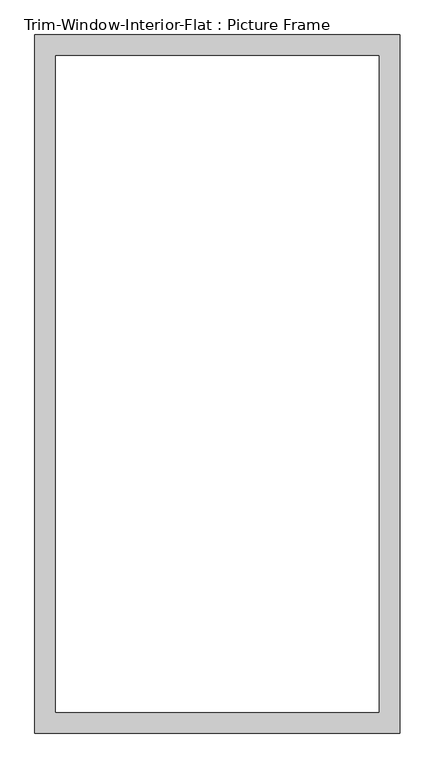
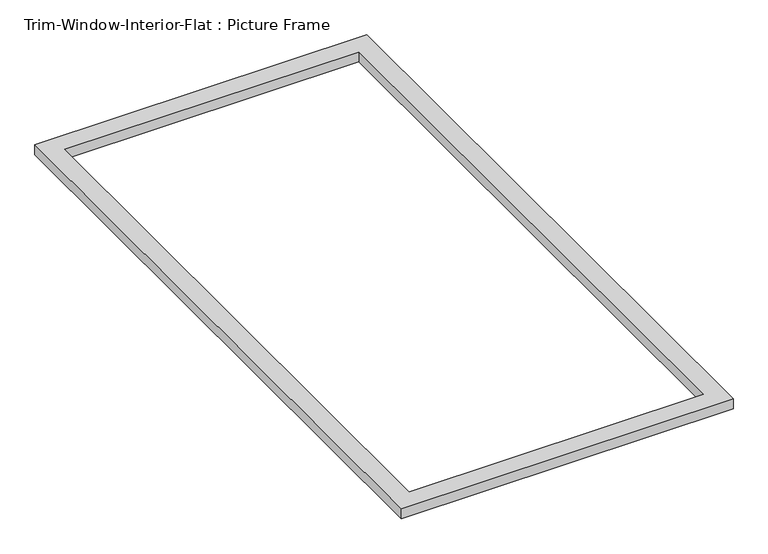
"""IFC4 building model written with IfcOpenShell, lengths in millimetres: proxy geometry, Trim-Window-Interior-Flat : Picture Frame."""

from ifc_helpers import new_model, si_unit, origin, origin_with_axes, place, context, project, spatial, polyline, outline, extrude, source, transform, mapped, element, save


def trim_window_interior_flat_picture_frame_a0ba83d5(model_context):
    return source(origin(), model_context, "Body", "SweptSolid", [
        extrude(outline(polyline([(501.65, -44.45), (-501.65, -44.45), (-501.65, 1873.25), (501.65, 1873.25), (501.65, -44.45)]), holes=[polyline([(444.5, 12.7), (444.5, 1816.1), (-444.5, 1816.1), (-444.5, 12.7), (444.5, 12.7)])]), origin_with_axes(), (0.0, 0.0, 1.0), 31.75),
    ])


if __name__ == "__main__":
    model = new_model("IFC4")
    model_context = context("Model", 3, world=origin())
    ifc_project = project(units=[si_unit("LENGTHUNIT", "METRE", prefix="MILLI")], contexts=[model_context])
    site = spatial("IfcSite", under=ifc_project)
    building = spatial("IfcBuilding", under=site)
    placement = place(None, origin())
    trim_window_interior_flat_picture_frame_shape = trim_window_interior_flat_picture_frame_a0ba83d5(model_context)
    element("IfcBuildingElementProxy", 1, Name="Trim-Window-Interior-Flat : Picture Frame", ObjectType="Trim-Window-Interior-Flat : Picture Frame", at=placement, inside=building, context=model_context, shape_type="MappedRepresentation", body=[
        mapped(trim_window_interior_flat_picture_frame_shape, transform((0.0, 0.0, 0.0), x_axis=(1.0, 0.0, 0.0), y_axis=(0.0, 1.0, 0.0), z_axis=(0.0, 0.0, 1.0))),
    ])
    save(model, "model.ifc")

# Revit data of these elements
# Type "Trim-Window-Interior-Flat : Picture Frame"
#   Trim Thickness_Picture Frame = 0' - 1 1/4"
#   Trim Width = 0' - 2 1/4"
#   Trim Thickness_with Sill = 0' - 0 3/4"
#   Sill Thickness = 0' - 1 1/4"
#   Opening Width [instance default] = 2' - 0"
#   Opening Height [instance default] = 3' - 0"
#   Default Elevation = 4' - 0"
#   Sill = no
#   Picture Frame = yes
#   Trim Material [instance default] = none
# Element 1 (IfcBuildingElementProxy, "Trim-Window-Interior-Flat : Picture Frame")
#   Opening Width = 3' - 0"
#   Opening Height = 6' - 0"
#   Trim Material = Wood - Stained
#   Materials on its faces: "Wood - Stained"
# Materials
#   "Wood - Stained": class "Wood", colour RGB 224 178 126, transparency 0, Cost = 0
